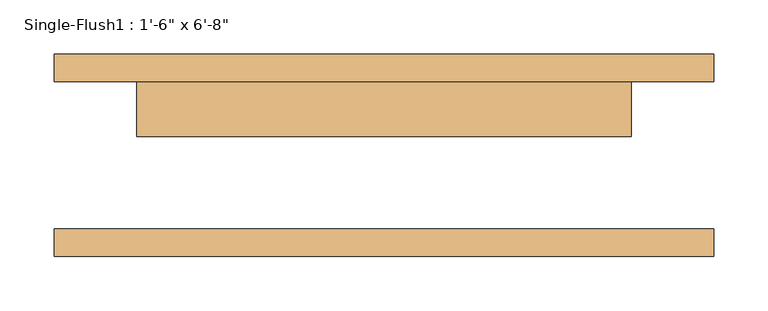
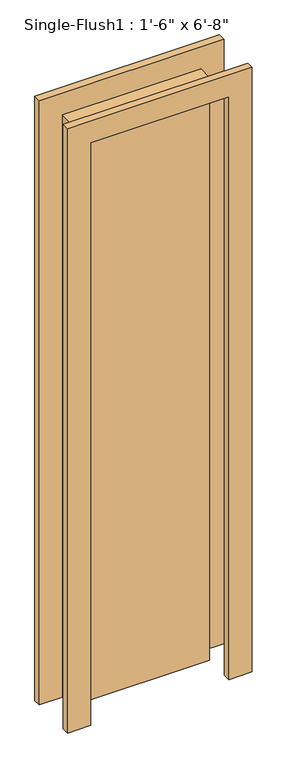
"""IFC4 building model written with IfcOpenShell, lengths in millimetres: door geometry."""

from ifc_helpers import new_model, si_unit, frame, origin, origin_with_axes, place, context, project, spatial, polyline, outline, extrude, source, transform, mapped, element, save


def door_c9619091(model_context):
    return source(origin(), model_context, "Body", "SweptSolid", [
        extrude(outline(polyline([(2108.2, -304.8), (0.0, -304.8), (0.0, -228.6), (2032.0, -228.6), (2032.0, 228.6), (0.0, 228.6), (0.0, 304.8), (2108.2, 304.8), (2108.2, -304.8)])), frame((0.0, 68.2625, 0.0), z_axis=(0.0, 1.0, 0.0), x_axis=(0.0, 0.0, 1.0)), (0.0, 0.0, 1.0), 25.4),
        extrude(outline(polyline([(2108.2, 304.8), (2108.2, -304.8), (0.0, -304.8), (0.0, -228.6), (2032.0, -228.6), (2032.0, 228.6), (0.0, 228.6), (0.0, 304.8), (2108.2, 304.8)])), frame((0.0, -93.6625, 0.0), z_axis=(0.0, 1.0, 0.0), x_axis=(0.0, 0.0, 1.0)), (0.0, 0.0, 1.0), 25.4),
        extrude(outline(polyline([(228.6, 17.4625), (-228.6, 17.4625), (-228.6, 68.2625), (228.6, 68.2625), (228.6, 17.4625)])), origin_with_axes(), (0.0, 0.0, 1.0), 2032.0),
    ])


if __name__ == "__main__":
    model = new_model("IFC4")
    model_context = context("Model", 3, world=origin())
    ifc_project = project(units=[si_unit("LENGTHUNIT", "METRE", prefix="MILLI")], contexts=[model_context])
    site = spatial("IfcSite", under=ifc_project)
    building = spatial("IfcBuilding", under=site)
    placement = place(None, origin())
    door_shape = door_c9619091(model_context)
    element("IfcDoor", 1, ObjectType="Single-Flush1 : 1'-6\" x 6'-8\"", at=placement, inside=building, context=model_context, shape_type="MappedRepresentation", body=[
        mapped(door_shape, transform((0.0, 0.0, 0.0), x_axis=(1.0, 0.0, 0.0), y_axis=(0.0, 1.0, 0.0), z_axis=(0.0, 0.0, 1.0))),
    ])
    save(model, "model.ifc")

# Revit data of these elements
# Type "Single-Flush1 : 1'-6\" x 6'-8\""
#   Type Mark = "24"
#   Construction Type Id = "MDOOR"
#   Assembly Code = "C1020"
#   Analytic Construction = "Metal"
#   Thickness = 0' - 2"
#   Heat Transfer Coefficient (U) = 3.7021 W/(m²·K)
#   Height = 6' - 8"
#   Trim Projection Ext = 0' - 1"
#   Trim Projection Int = 0' - 1"
#   Trim Width = 0' - 3"
#   Width = 1' - 6"
#   Door Material = Door - Panel
#   Frame Material = Door - Frame
#   Visual Light Transmittance = 0
#   Solar Heat Gain Coefficient = 0
#   Function = (empty or 0)
#   Wall Closure = (empty or 0)
# Element 1 (IfcDoor, "Single-Flush1 : 1'-6\" x 6'-8\"")
#   Materials on its faces: "Door - Frame", "Door - Panel"
# Materials
#   "Door - Panel": class "Wood", colour RGB 210 159 95, transparency 0, Cost = 0
#   "Door - Frame": class "Miscellaneous", colour RGB 118 70 51, transparency 0, Cost = 0
